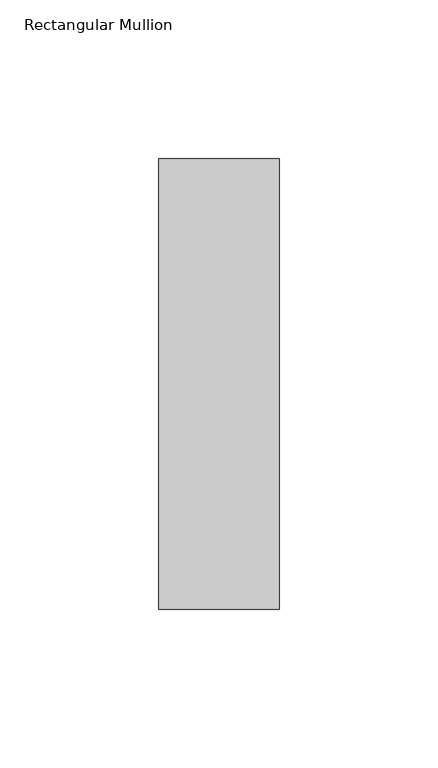
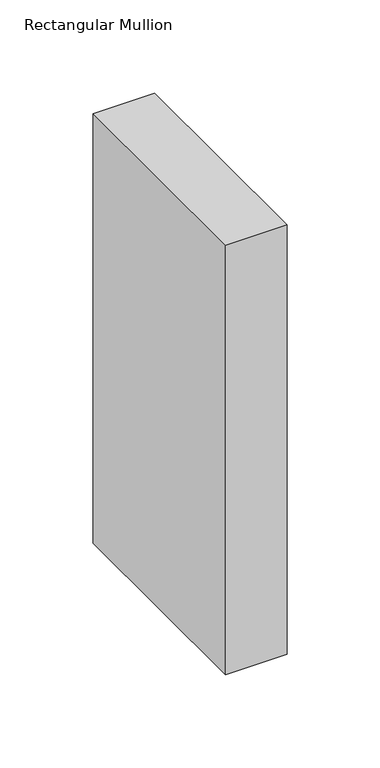
"""IFC4 building model written with IfcOpenShell, lengths in millimetres: member geometry, Rectangular Mullion : NLRS_21_CWM_hsb-regel 38x142_gen_rsf."""

from ifc_helpers import new_model, si_unit, frame, origin, place, context, project, spatial, polyline, outline, extrude, source, transform, mapped, element, save


def rectangular_mullion_baa0df26(model_context):
    return source(origin(), model_context, "Body", "SweptSolid", [
        extrude(outline(polyline([(-38.0, -71.0), (-38.0, 71.0), (0.0, 71.0), (0.0, -71.0), (-38.0, -71.0)])), frame((0.0, 0.0, -280.9999997), z_axis=(0.0, 0.0, 1.0), x_axis=(1.0, 0.0, 0.0)), (0.0, 0.0, 1.0), 280.9999997),
    ])


if __name__ == "__main__":
    model = new_model("IFC4")
    model_context = context("Model", 3, world=origin())
    ifc_project = project(units=[si_unit("LENGTHUNIT", "METRE", prefix="MILLI")], contexts=[model_context])
    site = spatial("IfcSite", under=ifc_project)
    building = spatial("IfcBuilding", under=site)
    placement = place(None, origin())
    rectangular_mullion_shape = rectangular_mullion_baa0df26(model_context)
    element("IfcMember", 1, ObjectType="Rectangular Mullion : NLRS_21_CWM_hsb-regel 38x142_gen_rsf", at=placement, inside=building, context=model_context, shape_type="MappedRepresentation", body=[
        mapped(rectangular_mullion_shape, transform((0.0, 0.0, 0.0), x_axis=(1.0, 0.0, 0.0), y_axis=(0.0, 1.0, 0.0), z_axis=(0.0, 0.0, 1.0))),
    ])
    save(model, "model.ifc")

# Revit data of these elements
# Type "Rectangular Mullion : NLRS_21_CWM_hsb-regel 38x142_gen_rsf"
#   Export Type to IFC As = "IfcWall"
#   Type IfcGUID = "07M7mRoiH1CR8m_RSKIwpF"
#   Assembly Code = "21.10"
#   built-in parameter 1007322 = 0.465879 (stored number, unit not read)
#   built-in parameter 1007321 = 0.062336 (stored number, unit not read)
#   built-in parameter 1007320 = 0.062336 (stored number, unit not read)
# Element 1 (IfcMember, "Rectangular Mullion : NLRS_21_CWM_hsb-regel 38x142_gen_rsf")
#   Materials on its faces: "NLRS_i2_hout naaldhout vuren_gen_rsf"
# Materials
#   "NLRS_i2_hout naaldhout vuren_gen_rsf": class "I - Hout", colour RGB 234 199 147, transparency 0, Keynote = "i2", Manufacturer = "Revit Standards Foundation", URL = "www.revitstandards.org", Description = "hout vuren", Cost = 0
